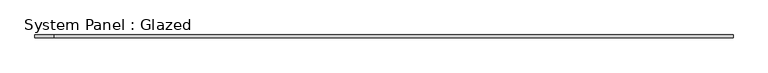
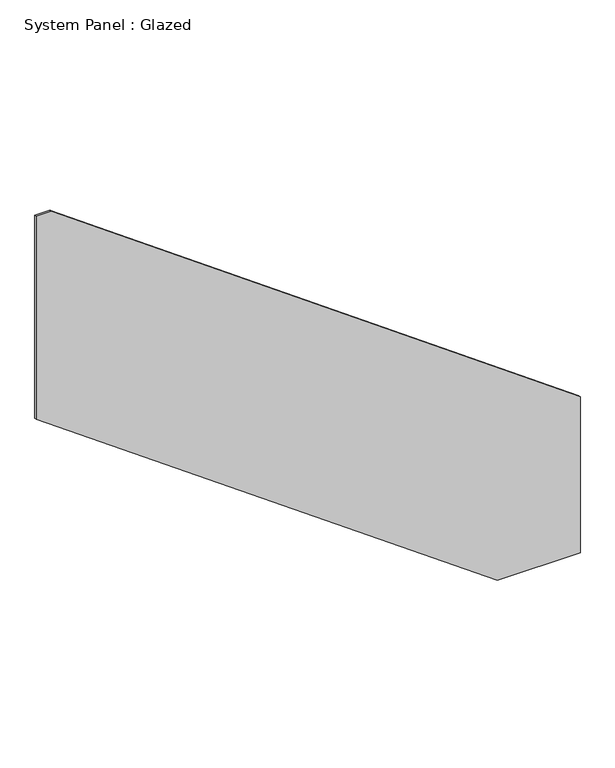
"""IFC4 building model written with IfcOpenShell, lengths in millimetres: plate geometry, System Panel : Glazed."""

from ifc_helpers import new_model, si_unit, frame, origin, place, context, project, spatial, polyline, outline, extrude, source, transform, mapped, element, save


def system_panel_glazed_bde8d024(model_context):
    return source(origin(), model_context, "Body", "SweptSolid", [
        extrude(outline(polyline([(0.0, 2300.7478333), (0.0, 3306.25), (2001.6508139, 3306.25), (6634.9240943, -3123.25), (6634.9240943, -3306.25), (4030.0, -3306.25), (0.0, 2300.7478333)])), frame((0.0, 24.5, 0.0), z_axis=(0.0, 1.0, 0.0), x_axis=(0.0, 0.0, 1.0)), (0.0, 0.0, 1.0), 25.0),
    ])


if __name__ == "__main__":
    model = new_model("IFC4")
    model_context = context("Model", 3, world=origin())
    ifc_project = project(units=[si_unit("LENGTHUNIT", "METRE", prefix="MILLI")], contexts=[model_context])
    site = spatial("IfcSite", under=ifc_project)
    building = spatial("IfcBuilding", under=site)
    placement = place(None, origin())
    system_panel_glazed_shape = system_panel_glazed_bde8d024(model_context)
    element("IfcPlate", 1, ObjectType="System Panel : Glazed", at=placement, inside=building, context=model_context, shape_type="MappedRepresentation", body=[
        mapped(system_panel_glazed_shape, transform((0.0, 0.0, 0.0), x_axis=(1.0, 0.0, 0.0), y_axis=(0.0, 1.0, 0.0), z_axis=(0.0, 0.0, 1.0))),
    ])
    save(model, "model.ifc")

# Revit data of these elements
# Type "System Panel : Glazed"
#   Keynote = "H11"
#   Construction Type Id = "GSP4R"
#   Analytic Construction = "1/8 in Pilkington single glazing"
#   Visual Light Transmittance = 0.9
#   Solar Heat Gain Coefficient = 0.86
#   Heat Transfer Coefficient (U) = 6.7069 W/(m²·K)
#   Define Thermal Properties by = 1
# Element 1 (IfcPlate, "System Panel : Glazed")
#   Materials on its faces: "Glass"
# Materials
#   "Glass": class "Glass", colour RGB 0 128 192, transparency 0.9, Description = "Soda Lime Glass", Cost = 0
